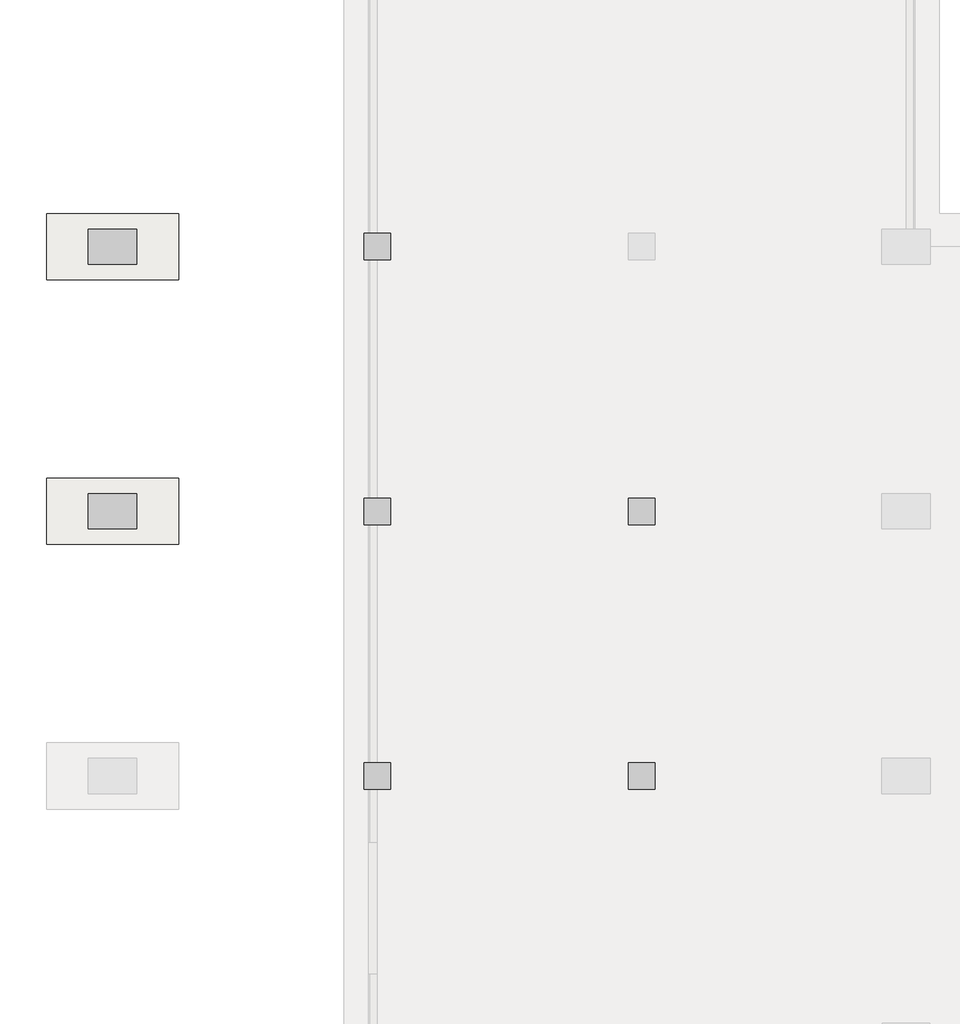
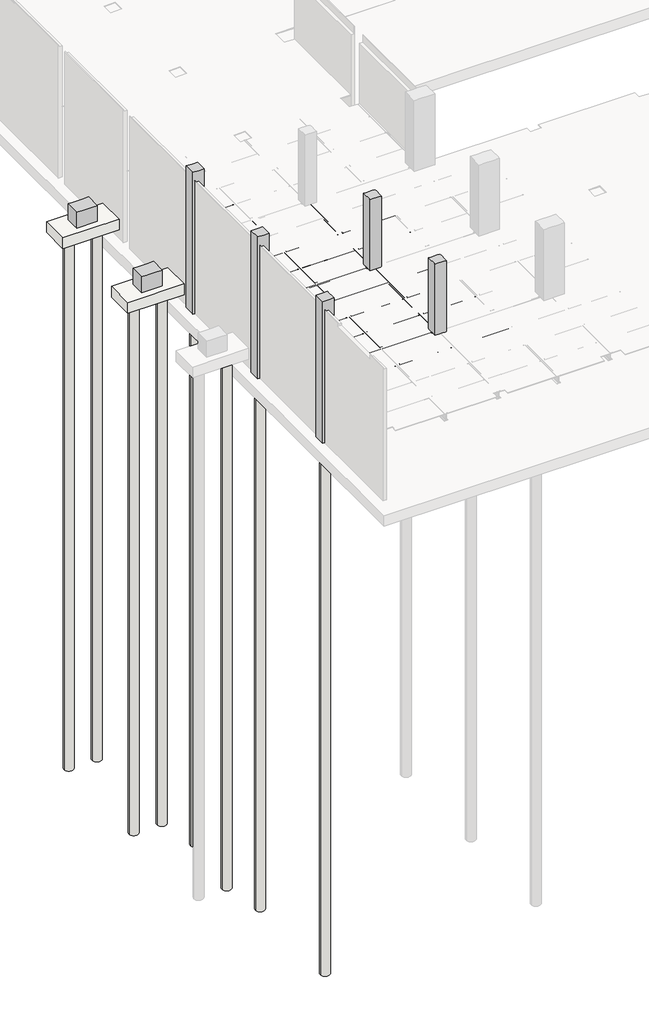
# Not in any storey, part 2 of 16: 26 beams, 10 slabs, 7 columns.
# Revit data of these elements (continued)
# Elements 3, 13 (IfcBeam, "Steel Framing_H_KS : H_SB_AR_S02_H-400x200x8x13_BSB1") (continued)
#   Materials on its faces: "Steel, 45-345"
# Elements 4, 5, 6, 7, 8, 9, 10, 14, 15, 16, 17, 18, 19, 20, 21, 22, 23, 24, 25, 26 (IfcBeam, "Steel Framing_C_KS : H_SB_AR_S02_C-150x75x6.5x10_J1")
#   Structural Material = Steel, 45-345
#   Phase Created = New Construction
#   Materials on its faces: "Steel, 45-345"
# Elements 27, 28 (IfcColumn, "RC_Column_Rectangular : H_SC_AR_S15_UG PED_Bit_800x1100_PD1")
#   Comments = ""
#   hec_material3 = none
#   hec_material2 = none
#   hec_material1 = none
#   Structural Material = 00_Concrete_Reinf. Conc.
#   Phase Created = New Construction
#   Materials on its faces: "00_Concrete_Reinf. Conc."
# Elements 29, 30, 31, 32, 33 (IfcColumn, "RC_Column_Rectangular : H_SC_AR_S15_UG PED_Bit_600x600_BC1")
#   Comments = ""
#   hec_material3 = none
#   hec_material2 = none
#   hec_material1 = none
#   Structural Material = 00_Concrete_Reinf. Conc.
#   Phase Created = New Construction
#   Materials on its faces: "00_Concrete_Reinf. Conc."
# Elements 34, 35 (IfcSlab, "Foundation Rectangular (Non-Pile) : H_SF_AR_S18_Shallow Fdn_Bitumen_1500x3000xT600_F1")
#   Comments = ""
#   Structural Material = 00_Concrete_Reinf. Conc.
#   Phase Created = New Construction
#   Materials on its faces: "00_Concrete_Reinf. Conc."
# Elements 36, 37, 38, 39, 40 (IfcSlab, "PILE : H_SF_AR_S19_PHC Pile_Pre-boring_D500_L30")
#   Structural Material = Concrete, Precast
#   Phase Created = New Construction
#   Materials on its faces: "Concrete, Precast"
# Elements 41, 42, 43 (IfcSlab, "PILE : H_SF_AR_S19_PHC Pile_Pre-boring_D500_L30")
#   Structural Material = none
#   Phase Created = New Construction
# Materials
#   "Steel, 45-345": class "Metal", colour RGB 189 187 185, transparency 0, Description = "Steel 345 MPa", Cost = 0
#   "00_Concrete_Reinf. Conc.": class "Concrete", colour RGB 176 176 176, transparency 0, Description = "Reinf. Conc.", Cost = 0, Image = Concrete.Cast-In-Place.Flat.Polished.Grey.jpg
#   "Concrete, Precast": class "Concrete", colour RGB 115 116 108, transparency 0, Description = "Precast concrete", Cost = 0
